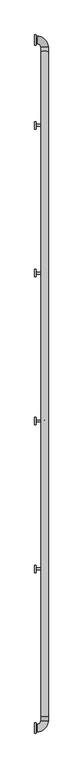
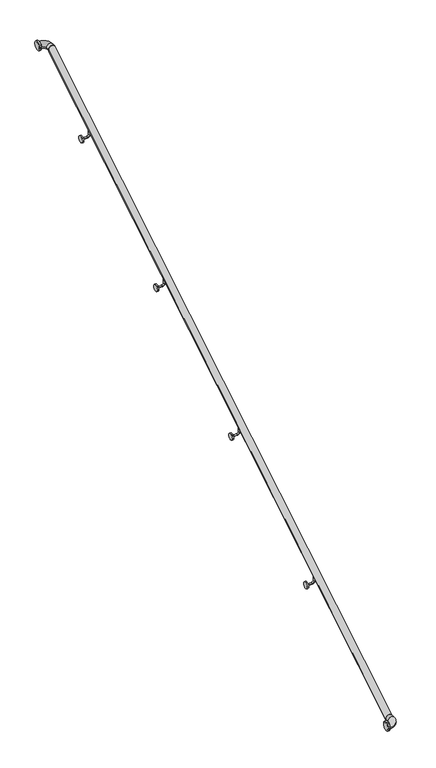
"""IFC4 building model written with IfcOpenShell, lengths in millimetres: railing geometry."""

from ifc_helpers import new_model, si_unit, point, frame, frame_2d, origin, place, context, project, spatial, circle_curve, ellipse_curve, trimmed, segment, composite_curve, outline, extrude, source, transform, mapped, element, save
from ifc_brep_helpers import plane_surface, cylinder_surface, revolved_surface, advanced_brep


def railing_eb7a726a(model_context):
    return source(origin(), model_context, "Body", "SolidModel", [
        advanced_brep(
        [(19158.0944438, 42249.3496945, 1051.653859), (19107.2944438, 42249.3496945, 1051.653859), (19158.0944438, 46749.3496945, 3771.653859), (19107.2944438, 46749.3496945, 3771.653859)],
        [
            (0, 1, ellipse_curve(frame((19132.6944438, 42249.3496945, 1051.653859), z_axis=(0.0, -1.0, 0.0), x_axis=(0.0, 0.0, -1.0)), 29.6794743, 25.4)),
            (1, 0, ellipse_curve(frame((19132.6944438, 42249.3496945, 1051.653859), z_axis=(0.0, -1.0, 0.0), x_axis=(0.0, 0.0, -1.0)), 29.6794743, 25.4)),
            (2, 3, ellipse_curve(frame((19132.6944438, 46749.3496945, 3771.653859), z_axis=(0.0, 1.0, 0.0), x_axis=(0.0, 0.0, -1.0)), 29.6794743, 25.4)),
            (3, 2, ellipse_curve(frame((19132.6944438, 46749.3496945, 3771.653859), z_axis=(0.0, 1.0, 0.0), x_axis=(0.0, 0.0, -1.0)), 29.6794743, 25.4)),
            (0, 2),
            (3, 1),
        ],
        [
            plane_surface(frame((19132.6944438, 42249.3496945, 1081.3333333), z_axis=(0.0, -1.0, 0.0), x_axis=(0.0, 0.0, 1.0))),
            plane_surface(frame((19132.6944438, 46749.3496945, 3801.3333333), z_axis=(0.0, 1.0, 0.0), x_axis=(0.0, 0.0, 1.0))),
            cylinder_surface(frame((19132.6944438, 42262.4888551, 1059.5957516), z_axis=(0.0, -0.8558103053667958, -0.5172897845772637), x_axis=(-1.0, 0.0, 0.0)), 25.4),
        ],
        [
            (0, [[1, 2]]),
            (1, [[3, 4]]),
            (2, [[-1, 5, -4, 6]]),
            (2, [[-2, -6, -3, -5]]),
        ],
    ),
        extrude(outline(composite_curve([segment(trimmed(circle_curve(frame_2d((46249.3496945, 3363.7521624)), 25.4), [point((46274.7496945, 3363.7521624))], [point((46223.9496945, 3363.7521624))], False, "CARTESIAN"), True, "CONTINUOUS"), segment(trimmed(circle_curve(frame_2d((46249.3496945, 3363.7521624)), 25.4), [point((46223.9496945, 3363.7521624))], [point((46274.7496945, 3363.7521624))], False, "CARTESIAN"), True, "CONTINUOUS")], self_intersect=False)), frame((19065.7444438, 0.0, 0.0), z_axis=(1.0, 0.0, 0.0), x_axis=(0.0, 1.0, 0.0)), (0.0, 0.0, 1.0), 9.525),
        advanced_brep(
        [(19132.7444438, 46242.9996945, 3439.7521624), (19132.7444438, 46255.6996945, 3439.7521624), (19132.7444438, 46255.6996945, 3382.8021624), (19132.7444438, 46242.9996945, 3382.8021624), (19113.6944438, 46255.6996945, 3363.7521624), (19113.6944438, 46242.9996945, 3363.7521624), (19075.2694438, 46242.9996945, 3363.7521624), (19075.2694438, 46255.6996945, 3363.7521624)],
        [
            (0, 1, circle_curve(frame((19132.7444438, 46249.3496945, 3439.7521624), z_axis=(0.0, 0.0, 1.0), x_axis=(0.0, 1.0, 0.0)), 6.35)),
            (1, 0, circle_curve(frame((19132.7444438, 46249.3496945, 3439.7521624), z_axis=(0.0, 0.0, 1.0), x_axis=(0.0, 1.0, 0.0)), 6.35)),
            (1, 2),
            (2, 3, circle_curve(frame((19132.7444438, 46249.3496945, 3382.8021624), z_axis=(0.0, 0.0, 1.0), x_axis=(0.0, 1.0, 0.0)), 6.35)),
            (3, 0),
            (3, 2, circle_curve(frame((19132.7444438, 46249.3496945, 3382.8021624), z_axis=(0.0, 0.0, 1.0), x_axis=(0.0, 1.0, 0.0)), 6.35)),
            (4, 5, circle_curve(frame((19113.6944438, 46249.3496945, 3363.7521624), z_axis=(1.0, 0.0, 0.0), x_axis=(0.0, 1.0, 0.0)), 6.35)),
            (5, 3, circle_curve(frame((19113.6944438, 46242.9996945, 3382.8021624), z_axis=(0.0, -1.0, 0.0), x_axis=(1.0, 0.0, 0.0)), 19.05)),
            (2, 4, circle_curve(frame((19113.6944438, 46255.6996945, 3382.8021624), z_axis=(0.0, 1.0, 0.0), x_axis=(1.0, 0.0, 0.0)), 19.05)),
            (5, 4, circle_curve(frame((19113.6944438, 46249.3496945, 3363.7521624), z_axis=(1.0, 0.0, 0.0), x_axis=(0.0, 1.0, 0.0)), 6.35)),
            (6, 7, circle_curve(frame((19075.2694438, 46249.3496945, 3363.7521624), z_axis=(-1.0, 0.0, 0.0), x_axis=(0.0, 1.0, 0.0)), 6.35)),
            (7, 6, circle_curve(frame((19075.2694438, 46249.3496945, 3363.7521624), z_axis=(-1.0, 0.0, 0.0), x_axis=(0.0, 1.0, 0.0)), 6.35)),
            (4, 7),
            (6, 5),
        ],
        [
            plane_surface(frame((19132.7444438, 46255.6996945, 3439.7521624), z_axis=(0.0, 0.0, 1.0), x_axis=(-1.0, 0.0, 0.0))),
            cylinder_surface(frame((19132.7444438, 46249.3496945, 3439.7521624), z_axis=(0.0, 0.0, 1.0), x_axis=(0.0, 1.0, 0.0)), 6.35),
            revolved_surface(trimmed(ellipse_curve(frame((19132.7444438, 46249.3496945, 3382.8021624), z_axis=(0.0, 0.0, -1.0), x_axis=(0.0, 1.0, 0.0)), 6.35, 6.35), [point((19132.7444438, 46242.9996945, 3382.8021624))], [point((19132.7444438, 46255.6996945, 3382.8021624))], True, "CARTESIAN"), (19113.6944438, 46249.3496945, 3382.8021624), (0.0, -1.0, 0.0)),
            revolved_surface(trimmed(ellipse_curve(frame((19132.7444438, 46249.3496945, 3382.8021624), z_axis=(0.0, 0.0, -1.0), x_axis=(0.0, 1.0, 0.0)), 6.35, 6.35), [point((19132.7444438, 46255.6996945, 3382.8021624))], [point((19132.7444438, 46242.9996945, 3382.8021624))], True, "CARTESIAN"), (19113.6944438, 46249.3496945, 3382.8021624), (0.0, -1.0, 0.0)),
            plane_surface(frame((19075.2694438, 46249.3496945, 3357.4021624), z_axis=(-1.0, 0.0, 0.0), x_axis=(0.0, 1.0, 0.0))),
            cylinder_surface(frame((19113.6944438, 46249.3496945, 3363.7521624), z_axis=(1.0, 0.0, 0.0), x_axis=(0.0, 1.0, 0.0)), 6.35),
        ],
        [
            (0, [[1, 2]]),
            (1, [[3, 4, 5, -2]]),
            (1, [[-5, 6, -3, -1]]),
            (2, [[7, 8, -4, 9]]),
            (3, [[10, -9, -6, -8]]),
            (4, [[11, 12]]),
            (5, [[13, -11, 14, -7]]),
            (5, [[-14, -12, -13, -10]]),
        ],
    ),
        extrude(outline(composite_curve([segment(trimmed(circle_curve(frame_2d((45249.3496945, 2759.307718)), 25.4), [point((45274.7496945, 2759.307718))], [point((45223.9496945, 2759.307718))], False, "CARTESIAN"), True, "CONTINUOUS"), segment(trimmed(circle_curve(frame_2d((45249.3496945, 2759.307718)), 25.4), [point((45223.9496945, 2759.307718))], [point((45274.7496945, 2759.307718))], False, "CARTESIAN"), True, "CONTINUOUS")], self_intersect=False)), frame((19065.7444438, 0.0, 0.0), z_axis=(1.0, 0.0, 0.0), x_axis=(0.0, 1.0, 0.0)), (0.0, 0.0, 1.0), 9.525),
        advanced_brep(
        [(19132.7444438, 45242.9996945, 2835.307718), (19132.7444438, 45255.6996945, 2835.307718), (19132.7444438, 45255.6996945, 2778.357718), (19132.7444438, 45242.9996945, 2778.357718), (19113.6944438, 45255.6996945, 2759.307718), (19113.6944438, 45242.9996945, 2759.307718), (19075.2694438, 45242.9996945, 2759.307718), (19075.2694438, 45255.6996945, 2759.307718)],
        [
            (0, 1, circle_curve(frame((19132.7444438, 45249.3496945, 2835.307718), z_axis=(0.0, 0.0, 1.0), x_axis=(0.0, 1.0, 0.0)), 6.35)),
            (1, 0, circle_curve(frame((19132.7444438, 45249.3496945, 2835.307718), z_axis=(0.0, 0.0, 1.0), x_axis=(0.0, 1.0, 0.0)), 6.35)),
            (1, 2),
            (2, 3, circle_curve(frame((19132.7444438, 45249.3496945, 2778.357718), z_axis=(0.0, 0.0, 1.0), x_axis=(0.0, 1.0, 0.0)), 6.35)),
            (3, 0),
            (3, 2, circle_curve(frame((19132.7444438, 45249.3496945, 2778.357718), z_axis=(0.0, 0.0, 1.0), x_axis=(0.0, 1.0, 0.0)), 6.35)),
            (4, 5, circle_curve(frame((19113.6944438, 45249.3496945, 2759.307718), z_axis=(1.0, 0.0, 0.0), x_axis=(0.0, 1.0, 0.0)), 6.35)),
            (5, 3, circle_curve(frame((19113.6944438, 45242.9996945, 2778.357718), z_axis=(0.0, -1.0, 0.0), x_axis=(1.0, 0.0, 0.0)), 19.05)),
            (2, 4, circle_curve(frame((19113.6944438, 45255.6996945, 2778.357718), z_axis=(0.0, 1.0, 0.0), x_axis=(1.0, 0.0, 0.0)), 19.05)),
            (5, 4, circle_curve(frame((19113.6944438, 45249.3496945, 2759.307718), z_axis=(1.0, 0.0, 0.0), x_axis=(0.0, 1.0, 0.0)), 6.35)),
            (6, 7, circle_curve(frame((19075.2694438, 45249.3496945, 2759.307718), z_axis=(-1.0, 0.0, 0.0), x_axis=(0.0, 1.0, 0.0)), 6.35)),
            (7, 6, circle_curve(frame((19075.2694438, 45249.3496945, 2759.307718), z_axis=(-1.0, 0.0, 0.0), x_axis=(0.0, 1.0, 0.0)), 6.35)),
            (4, 7),
            (6, 5),
        ],
        [
            plane_surface(frame((19132.7444438, 45255.6996945, 2835.307718), z_axis=(0.0, 0.0, 1.0), x_axis=(-1.0, 0.0, 0.0))),
            cylinder_surface(frame((19132.7444438, 45249.3496945, 2835.307718), z_axis=(0.0, 0.0, 1.0), x_axis=(0.0, 1.0, 0.0)), 6.35),
            revolved_surface(trimmed(ellipse_curve(frame((19132.7444438, 45249.3496945, 2778.357718), z_axis=(0.0, 0.0, -1.0), x_axis=(0.0, 1.0, 0.0)), 6.35, 6.35), [point((19132.7444438, 45242.9996945, 2778.357718))], [point((19132.7444438, 45255.6996945, 2778.357718))], True, "CARTESIAN"), (19113.6944438, 45249.3496945, 2778.357718), (0.0, -1.0, 0.0)),
            revolved_surface(trimmed(ellipse_curve(frame((19132.7444438, 45249.3496945, 2778.357718), z_axis=(0.0, 0.0, -1.0), x_axis=(0.0, 1.0, 0.0)), 6.35, 6.35), [point((19132.7444438, 45255.6996945, 2778.357718))], [point((19132.7444438, 45242.9996945, 2778.357718))], True, "CARTESIAN"), (19113.6944438, 45249.3496945, 2778.357718), (0.0, -1.0, 0.0)),
            plane_surface(frame((19075.2694438, 45249.3496945, 2752.957718), z_axis=(-1.0, 0.0, 0.0), x_axis=(0.0, 1.0, 0.0))),
            cylinder_surface(frame((19113.6944438, 45249.3496945, 2759.307718), z_axis=(1.0, 0.0, 0.0), x_axis=(0.0, 1.0, 0.0)), 6.35),
        ],
        [
            (0, [[1, 2]]),
            (1, [[3, 4, 5, -2]]),
            (1, [[-5, 6, -3, -1]]),
            (2, [[7, 8, -4, 9]]),
            (3, [[10, -9, -6, -8]]),
            (4, [[11, 12]]),
            (5, [[13, -11, 14, -7]]),
            (5, [[-14, -12, -13, -10]]),
        ],
    ),
        extrude(outline(composite_curve([segment(trimmed(circle_curve(frame_2d((44249.3496945, 2154.8632735)), 25.4), [point((44274.7496945, 2154.8632735))], [point((44223.9496945, 2154.8632735))], False, "CARTESIAN"), True, "CONTINUOUS"), segment(trimmed(circle_curve(frame_2d((44249.3496945, 2154.8632735)), 25.4), [point((44223.9496945, 2154.8632735))], [point((44274.7496945, 2154.8632735))], False, "CARTESIAN"), True, "CONTINUOUS")], self_intersect=False)), frame((19065.7444438, 0.0, 0.0), z_axis=(1.0, 0.0, 0.0), x_axis=(0.0, 1.0, 0.0)), (0.0, 0.0, 1.0), 9.525),
        advanced_brep(
        [(19132.7444438, 44242.9996945, 2230.8632735), (19132.7444438, 44255.6996945, 2230.8632735), (19132.7444438, 44255.6996945, 2173.9132735), (19132.7444438, 44242.9996945, 2173.9132735), (19113.6944438, 44255.6996945, 2154.8632735), (19113.6944438, 44242.9996945, 2154.8632735), (19075.2694438, 44242.9996945, 2154.8632735), (19075.2694438, 44255.6996945, 2154.8632735)],
        [
            (0, 1, circle_curve(frame((19132.7444438, 44249.3496945, 2230.8632735), z_axis=(0.0, 0.0, 1.0), x_axis=(0.0, 1.0, 0.0)), 6.35)),
            (1, 0, circle_curve(frame((19132.7444438, 44249.3496945, 2230.8632735), z_axis=(0.0, 0.0, 1.0), x_axis=(0.0, 1.0, 0.0)), 6.35)),
            (1, 2),
            (2, 3, circle_curve(frame((19132.7444438, 44249.3496945, 2173.9132735), z_axis=(0.0, 0.0, 1.0), x_axis=(0.0, 1.0, 0.0)), 6.35)),
            (3, 0),
            (3, 2, circle_curve(frame((19132.7444438, 44249.3496945, 2173.9132735), z_axis=(0.0, 0.0, 1.0), x_axis=(0.0, 1.0, 0.0)), 6.35)),
            (4, 5, circle_curve(frame((19113.6944438, 44249.3496945, 2154.8632735), z_axis=(1.0, 0.0, 0.0), x_axis=(0.0, 1.0, 0.0)), 6.35)),
            (5, 3, circle_curve(frame((19113.6944438, 44242.9996945, 2173.9132735), z_axis=(0.0, -1.0, 0.0), x_axis=(1.0, 0.0, 0.0)), 19.05)),
            (2, 4, circle_curve(frame((19113.6944438, 44255.6996945, 2173.9132735), z_axis=(0.0, 1.0, 0.0), x_axis=(1.0, 0.0, 0.0)), 19.05)),
            (5, 4, circle_curve(frame((19113.6944438, 44249.3496945, 2154.8632735), z_axis=(1.0, 0.0, 0.0), x_axis=(0.0, 1.0, 0.0)), 6.35)),
            (6, 7, circle_curve(frame((19075.2694438, 44249.3496945, 2154.8632735), z_axis=(-1.0, 0.0, 0.0), x_axis=(0.0, 1.0, 0.0)), 6.35)),
            (7, 6, circle_curve(frame((19075.2694438, 44249.3496945, 2154.8632735), z_axis=(-1.0, 0.0, 0.0), x_axis=(0.0, 1.0, 0.0)), 6.35)),
            (4, 7),
            (6, 5),
        ],
        [
            plane_surface(frame((19132.7444438, 44255.6996945, 2230.8632735), z_axis=(0.0, 0.0, 1.0), x_axis=(-1.0, 0.0, 0.0))),
            cylinder_surface(frame((19132.7444438, 44249.3496945, 2230.8632735), z_axis=(0.0, 0.0, 1.0), x_axis=(0.0, 1.0, 0.0)), 6.35),
            revolved_surface(trimmed(ellipse_curve(frame((19132.7444438, 44249.3496945, 2173.9132735), z_axis=(0.0, 0.0, -1.0), x_axis=(0.0, 1.0, 0.0)), 6.35, 6.35), [point((19132.7444438, 44242.9996945, 2173.9132735))], [point((19132.7444438, 44255.6996945, 2173.9132735))], True, "CARTESIAN"), (19113.6944438, 44249.3496945, 2173.9132735), (0.0, -1.0, 0.0)),
            revolved_surface(trimmed(ellipse_curve(frame((19132.7444438, 44249.3496945, 2173.9132735), z_axis=(0.0, 0.0, -1.0), x_axis=(0.0, 1.0, 0.0)), 6.35, 6.35), [point((19132.7444438, 44255.6996945, 2173.9132735))], [point((19132.7444438, 44242.9996945, 2173.9132735))], True, "CARTESIAN"), (19113.6944438, 44249.3496945, 2173.9132735), (0.0, -1.0, 0.0)),
            plane_surface(frame((19075.2694438, 44249.3496945, 2148.5132735), z_axis=(-1.0, 0.0, 0.0), x_axis=(0.0, 1.0, 0.0))),
            cylinder_surface(frame((19113.6944438, 44249.3496945, 2154.8632735), z_axis=(1.0, 0.0, 0.0), x_axis=(0.0, 1.0, 0.0)), 6.35),
        ],
        [
            (0, [[1, 2]]),
            (1, [[3, 4, 5, -2]]),
            (1, [[-5, 6, -3, -1]]),
            (2, [[7, 8, -4, 9]]),
            (3, [[10, -9, -6, -8]]),
            (4, [[11, 12]]),
            (5, [[13, -11, 14, -7]]),
            (5, [[-14, -12, -13, -10]]),
        ],
    ),
        extrude(outline(composite_curve([segment(trimmed(circle_curve(frame_2d((43249.3496945, 1550.4188291)), 25.4), [point((43274.7496945, 1550.4188291))], [point((43223.9496945, 1550.4188291))], False, "CARTESIAN"), True, "CONTINUOUS"), segment(trimmed(circle_curve(frame_2d((43249.3496945, 1550.4188291)), 25.4), [point((43223.9496945, 1550.4188291))], [point((43274.7496945, 1550.4188291))], False, "CARTESIAN"), True, "CONTINUOUS")], self_intersect=False)), frame((19065.7444438, 0.0, 0.0), z_axis=(1.0, 0.0, 0.0), x_axis=(0.0, 1.0, 0.0)), (0.0, 0.0, 1.0), 9.525),
        advanced_brep(
        [(19132.7444438, 43242.9996945, 1626.4188291), (19132.7444438, 43255.6996945, 1626.4188291), (19132.7444438, 43255.6996945, 1569.4688291), (19132.7444438, 43242.9996945, 1569.4688291), (19113.6944438, 43255.6996945, 1550.4188291), (19113.6944438, 43242.9996945, 1550.4188291), (19075.2694438, 43242.9996945, 1550.4188291), (19075.2694438, 43255.6996945, 1550.4188291)],
        [
            (0, 1, circle_curve(frame((19132.7444438, 43249.3496945, 1626.4188291), z_axis=(0.0, 0.0, 1.0), x_axis=(0.0, 1.0, 0.0)), 6.35)),
            (1, 0, circle_curve(frame((19132.7444438, 43249.3496945, 1626.4188291), z_axis=(0.0, 0.0, 1.0), x_axis=(0.0, 1.0, 0.0)), 6.35)),
            (1, 2),
            (2, 3, circle_curve(frame((19132.7444438, 43249.3496945, 1569.4688291), z_axis=(0.0, 0.0, 1.0), x_axis=(0.0, 1.0, 0.0)), 6.35)),
            (3, 0),
            (3, 2, circle_curve(frame((19132.7444438, 43249.3496945, 1569.4688291), z_axis=(0.0, 0.0, 1.0), x_axis=(0.0, 1.0, 0.0)), 6.35)),
            (4, 5, circle_curve(frame((19113.6944438, 43249.3496945, 1550.4188291), z_axis=(1.0, 0.0, 0.0), x_axis=(0.0, 1.0, 0.0)), 6.35)),
            (5, 3, circle_curve(frame((19113.6944438, 43242.9996945, 1569.4688291), z_axis=(0.0, -1.0, 0.0), x_axis=(1.0, 0.0, 0.0)), 19.05)),
            (2, 4, circle_curve(frame((19113.6944438, 43255.6996945, 1569.4688291), z_axis=(0.0, 1.0, 0.0), x_axis=(1.0, 0.0, 0.0)), 19.05)),
            (5, 4, circle_curve(frame((19113.6944438, 43249.3496945, 1550.4188291), z_axis=(1.0, 0.0, 0.0), x_axis=(0.0, 1.0, 0.0)), 6.35)),
            (6, 7, circle_curve(frame((19075.2694438, 43249.3496945, 1550.4188291), z_axis=(-1.0, 0.0, 0.0), x_axis=(0.0, 1.0, 0.0)), 6.35)),
            (7, 6, circle_curve(frame((19075.2694438, 43249.3496945, 1550.4188291), z_axis=(-1.0, 0.0, 0.0), x_axis=(0.0, 1.0, 0.0)), 6.35)),
            (4, 7),
            (6, 5),
        ],
        [
            plane_surface(frame((19132.7444438, 43255.6996945, 1626.4188291), z_axis=(0.0, 0.0, 1.0), x_axis=(-1.0, 0.0, 0.0))),
            cylinder_surface(frame((19132.7444438, 43249.3496945, 1626.4188291), z_axis=(0.0, 0.0, 1.0), x_axis=(0.0, 1.0, 0.0)), 6.35),
            revolved_surface(trimmed(ellipse_curve(frame((19132.7444438, 43249.3496945, 1569.4688291), z_axis=(0.0, 0.0, -1.0), x_axis=(0.0, 1.0, 0.0)), 6.35, 6.35), [point((19132.7444438, 43242.9996945, 1569.4688291))], [point((19132.7444438, 43255.6996945, 1569.4688291))], True, "CARTESIAN"), (19113.6944438, 43249.3496945, 1569.4688291), (0.0, -1.0, 0.0)),
            revolved_surface(trimmed(ellipse_curve(frame((19132.7444438, 43249.3496945, 1569.4688291), z_axis=(0.0, 0.0, -1.0), x_axis=(0.0, 1.0, 0.0)), 6.35, 6.35), [point((19132.7444438, 43255.6996945, 1569.4688291))], [point((19132.7444438, 43242.9996945, 1569.4688291))], True, "CARTESIAN"), (19113.6944438, 43249.3496945, 1569.4688291), (0.0, -1.0, 0.0)),
            plane_surface(frame((19075.2694438, 43249.3496945, 1544.0688291), z_axis=(-1.0, 0.0, 0.0), x_axis=(0.0, 1.0, 0.0))),
            cylinder_surface(frame((19113.6944438, 43249.3496945, 1550.4188291), z_axis=(1.0, 0.0, 0.0), x_axis=(0.0, 1.0, 0.0)), 6.35),
        ],
        [
            (0, [[1, 2]]),
            (1, [[3, 4, 5, -2]]),
            (1, [[-5, 6, -3, -1]]),
            (2, [[7, 8, -4, 9]]),
            (3, [[10, -9, -6, -8]]),
            (4, [[11, 12]]),
            (5, [[13, -11, 14, -7]]),
            (5, [[-14, -12, -13, -10]]),
        ],
    ),
        extrude(outline(composite_curve([segment(trimmed(circle_curve(frame_2d((46825.3496945, 3776.0333333)), 35.4), [point((46860.7496945, 3776.0333333))], [point((46789.9496945, 3776.0333333))], False, "CARTESIAN"), True, "CONTINUOUS"), segment(trimmed(circle_curve(frame_2d((46825.3496945, 3776.0333333)), 35.4), [point((46789.9496945, 3776.0333333))], [point((46860.7496945, 3776.0333333))], False, "CARTESIAN"), True, "CONTINUOUS")], self_intersect=False)), frame((19065.7444438, 0.0, 0.0), z_axis=(1.0, 0.0, 0.0), x_axis=(0.0, 1.0, 0.0)), (0.0, 0.0, 1.0), 9.525),
        advanced_brep(
        [(19107.3444438, 46749.3496945, 3776.0333333), (19158.1444438, 46749.3496945, 3776.0333333), (19158.1444438, 46776.8496945, 3776.0333333), (19107.3444438, 46776.8496945, 3776.0333333), (19084.2444438, 46850.7496945, 3776.0333333), (19084.2444438, 46799.9496945, 3776.0333333), (19065.7444438, 46799.9496945, 3776.0333333), (19065.7444438, 46850.7496945, 3776.0333333)],
        [
            (0, 1, circle_curve(frame((19132.7444438, 46749.3496945, 3776.0333333), z_axis=(0.0, -1.0, 0.0), x_axis=(1.0, 0.0, 0.0)), 25.4)),
            (1, 0, circle_curve(frame((19132.7444438, 46749.3496945, 3776.0333333), z_axis=(0.0, -1.0, 0.0), x_axis=(1.0, 0.0, 0.0)), 25.4)),
            (1, 2),
            (2, 3, circle_curve(frame((19132.7444438, 46776.8496945, 3776.0333333), z_axis=(0.0, -1.0, 0.0), x_axis=(1.0, 0.0, 0.0)), 25.4)),
            (3, 0),
            (3, 2, circle_curve(frame((19132.7444438, 46776.8496945, 3776.0333333), z_axis=(0.0, -1.0, 0.0), x_axis=(1.0, 0.0, 0.0)), 25.4)),
            (4, 5, circle_curve(frame((19084.2444438, 46825.3496945, 3776.0333333), z_axis=(1.0, 0.0, 0.0), x_axis=(0.0, 1.0, 0.0)), 25.4)),
            (5, 3, circle_curve(frame((19084.2444438, 46776.8496945, 3776.0333333), z_axis=(0.0, 0.0, -1.0), x_axis=(1.0, 0.0, 0.0)), 23.1)),
            (2, 4, circle_curve(frame((19084.2444438, 46776.8496945, 3776.0333333), z_axis=(0.0, 0.0, 1.0), x_axis=(1.0, 0.0, 0.0)), 73.9)),
            (5, 4, circle_curve(frame((19084.2444438, 46825.3496945, 3776.0333333), z_axis=(1.0, 0.0, 0.0), x_axis=(0.0, 1.0, 0.0)), 25.4)),
            (6, 7, circle_curve(frame((19065.7444438, 46825.3496945, 3776.0333333), z_axis=(-1.0, 0.0, 0.0), x_axis=(0.0, 1.0, 0.0)), 25.4)),
            (7, 6, circle_curve(frame((19065.7444438, 46825.3496945, 3776.0333333), z_axis=(-1.0, 0.0, 0.0), x_axis=(0.0, 1.0, 0.0)), 25.4)),
            (4, 7),
            (6, 5),
        ],
        [
            plane_surface(frame((19132.7444438, 46749.3496945, 3776.0333333), z_axis=(0.0, -1.0, 0.0), x_axis=(0.0, 0.0, 1.0))),
            cylinder_surface(frame((19132.7444438, 46749.3496945, 3776.0333333), z_axis=(0.0, -1.0, 0.0), x_axis=(1.0, 0.0, 0.0)), 25.4),
            revolved_surface(trimmed(ellipse_curve(frame((19132.7444438, 46776.8496945, 3776.0333333), z_axis=(0.0, 1.0, 0.0), x_axis=(1.0, 0.0, 0.0)), 25.4, 25.4), [point((19107.3444438, 46776.8496945, 3776.0333333))], [point((19158.1444438, 46776.8496945, 3776.0333333))], True, "CARTESIAN"), (19084.2444438, 46776.8496945, 3776.0333333), (0.0, 0.0, -1.0)),
            revolved_surface(trimmed(ellipse_curve(frame((19132.7444438, 46776.8496945, 3776.0333333), z_axis=(0.0, 1.0, 0.0), x_axis=(1.0, 0.0, 0.0)), 25.4, 25.4), [point((19158.1444438, 46776.8496945, 3776.0333333))], [point((19107.3444438, 46776.8496945, 3776.0333333))], True, "CARTESIAN"), (19084.2444438, 46776.8496945, 3776.0333333), (0.0, 0.0, -1.0)),
            plane_surface(frame((19065.7444438, 46825.3496945, 3776.0333333), z_axis=(-1.0, 0.0, 0.0), x_axis=(0.0, 0.0, 1.0))),
            cylinder_surface(frame((19084.2444438, 46825.3496945, 3776.0333333), z_axis=(1.0, 0.0, 0.0), x_axis=(0.0, 1.0, 0.0)), 25.4),
        ],
        [
            (0, [[1, 2]]),
            (1, [[3, 4, 5, -2]]),
            (1, [[-5, 6, -3, -1]]),
            (2, [[7, 8, -4, 9]]),
            (3, [[10, -9, -6, -8]]),
            (4, [[11, 12]]),
            (5, [[13, -11, 14, -7]]),
            (5, [[-14, -12, -13, -10]]),
        ],
    ),
        extrude(outline(composite_curve([segment(trimmed(circle_curve(frame_2d((42173.3496945, 1056.0333333)), 35.4), [point((42208.7496945, 1056.0333333))], [point((42137.9496945, 1056.0333333))], False, "CARTESIAN"), True, "CONTINUOUS"), segment(trimmed(circle_curve(frame_2d((42173.3496945, 1056.0333333)), 35.4), [point((42137.9496945, 1056.0333333))], [point((42208.7496945, 1056.0333333))], False, "CARTESIAN"), True, "CONTINUOUS")], self_intersect=False)), frame((19065.7444438, 0.0, 0.0), z_axis=(1.0, 0.0, 0.0), x_axis=(0.0, 1.0, 0.0)), (0.0, 0.0, 1.0), 9.525),
        advanced_brep(
        [(19158.1444438, 42249.3496945, 1056.0333333), (19107.3444438, 42249.3496945, 1056.0333333), (19158.1444438, 42221.8496945, 1056.0333333), (19107.3444438, 42221.8496945, 1056.0333333), (19084.2444438, 42147.9496945, 1056.0333333), (19084.2444438, 42198.7496945, 1056.0333333), (19065.7444438, 42147.9496945, 1056.0333333), (19065.7444438, 42198.7496945, 1056.0333333)],
        [
            (0, 1, circle_curve(frame((19132.7444438, 42249.3496945, 1056.0333333), z_axis=(0.0, 1.0, 0.0), x_axis=(-1.0, 0.0, 0.0)), 25.4)),
            (1, 0, circle_curve(frame((19132.7444438, 42249.3496945, 1056.0333333), z_axis=(0.0, 1.0, 0.0), x_axis=(-1.0, 0.0, 0.0)), 25.4)),
            (0, 2),
            (2, 3, circle_curve(frame((19132.7444438, 42221.8496945, 1056.0333333), z_axis=(0.0, 1.0, 0.0), x_axis=(-1.0, 0.0, 0.0)), 25.4)),
            (3, 1),
            (3, 2, circle_curve(frame((19132.7444438, 42221.8496945, 1056.0333333), z_axis=(0.0, 1.0, 0.0), x_axis=(-1.0, 0.0, 0.0)), 25.4)),
            (4, 5, circle_curve(frame((19084.2444438, 42173.3496945, 1056.0333333), z_axis=(1.0, 0.0, 0.0), x_axis=(0.0, 1.0, 0.0)), 25.4)),
            (5, 3, circle_curve(frame((19084.2444438, 42221.8496945, 1056.0333333), z_axis=(0.0, 0.0, 1.0), x_axis=(1.0, 0.0, 0.0)), 23.1)),
            (2, 4, circle_curve(frame((19084.2444438, 42221.8496945, 1056.0333333), z_axis=(0.0, 0.0, -1.0), x_axis=(1.0, 0.0, 0.0)), 73.9)),
            (5, 4, circle_curve(frame((19084.2444438, 42173.3496945, 1056.0333333), z_axis=(1.0, 0.0, 0.0), x_axis=(0.0, 1.0, 0.0)), 25.4)),
            (6, 7, circle_curve(frame((19065.7444438, 42173.3496945, 1056.0333333), z_axis=(-1.0, 0.0, 0.0), x_axis=(0.0, 1.0, 0.0)), 25.4)),
            (7, 6, circle_curve(frame((19065.7444438, 42173.3496945, 1056.0333333), z_axis=(-1.0, 0.0, 0.0), x_axis=(0.0, 1.0, 0.0)), 25.4)),
            (4, 6),
            (7, 5),
        ],
        [
            plane_surface(frame((19132.7444438, 42249.3496945, 1056.0333333), z_axis=(0.0, 1.0, 0.0), x_axis=(0.0, 0.0, 1.0))),
            cylinder_surface(frame((19132.7444438, 42249.3496945, 1056.0333333), z_axis=(0.0, 1.0, 0.0), x_axis=(-1.0, 0.0, 0.0)), 25.4),
            revolved_surface(trimmed(ellipse_curve(frame((19132.7444438, 42221.8496945, 1056.0333333), z_axis=(0.0, -1.0, 0.0), x_axis=(-1.0, 0.0, 0.0)), 25.4, 25.4), [point((19107.3444438, 42221.8496945, 1056.0333333))], [point((19158.1444438, 42221.8496945, 1056.0333333))], True, "CARTESIAN"), (19084.2444438, 42221.8496945, 1056.0333333), (0.0, 0.0, 1.0)),
            revolved_surface(trimmed(ellipse_curve(frame((19132.7444438, 42221.8496945, 1056.0333333), z_axis=(0.0, -1.0, 0.0), x_axis=(-1.0, 0.0, 0.0)), 25.4, 25.4), [point((19158.1444438, 42221.8496945, 1056.0333333))], [point((19107.3444438, 42221.8496945, 1056.0333333))], True, "CARTESIAN"), (19084.2444438, 42221.8496945, 1056.0333333), (0.0, 0.0, 1.0)),
            plane_surface(frame((19065.7444438, 42173.3496945, 1056.0333333), z_axis=(-1.0, 0.0, 0.0), x_axis=(0.0, 0.0, 1.0))),
            cylinder_surface(frame((19084.2444438, 42173.3496945, 1056.0333333), z_axis=(1.0, 0.0, 0.0), x_axis=(0.0, 1.0, 0.0)), 25.4),
        ],
        [
            (0, [[1, 2]]),
            (1, [[3, 4, 5, -1]]),
            (1, [[-5, 6, -3, -2]]),
            (2, [[7, 8, -4, 9]]),
            (3, [[10, -9, -6, -8]]),
            (4, [[11, 12]]),
            (5, [[13, -12, 14, -7]]),
            (5, [[-14, -11, -13, -10]]),
        ],
    ),
    ])


if __name__ == "__main__":
    model = new_model("IFC4")
    model_context = context("Model", 3, world=origin())
    ifc_project = project(units=[si_unit("LENGTHUNIT", "METRE", prefix="MILLI")], contexts=[model_context])
    site = spatial("IfcSite", under=ifc_project)
    building = spatial("IfcBuilding", under=site)
    placement = place(None, origin())
    railing_shape = railing_eb7a726a(model_context)
    element("IfcRailing", 1, at=placement, inside=building, context=model_context, shape_type="MappedRepresentation", body=[
        mapped(railing_shape, transform((0.0, 0.0, 0.0), x_axis=(1.0, 0.0, 0.0), y_axis=(0.0, 1.0, 0.0), z_axis=(0.0, 0.0, 1.0))),
    ])
    save(model, "model.ifc")

# Revit data of these elements
# Element 1 (IfcRailing)
#   Materials on its faces: "Ferro - Pintura Esmalte"
# Materials
#   "Ferro - Pintura Esmalte": class "Pintura", colour RGB 255 255 255, transparency 0, Cost = 0
